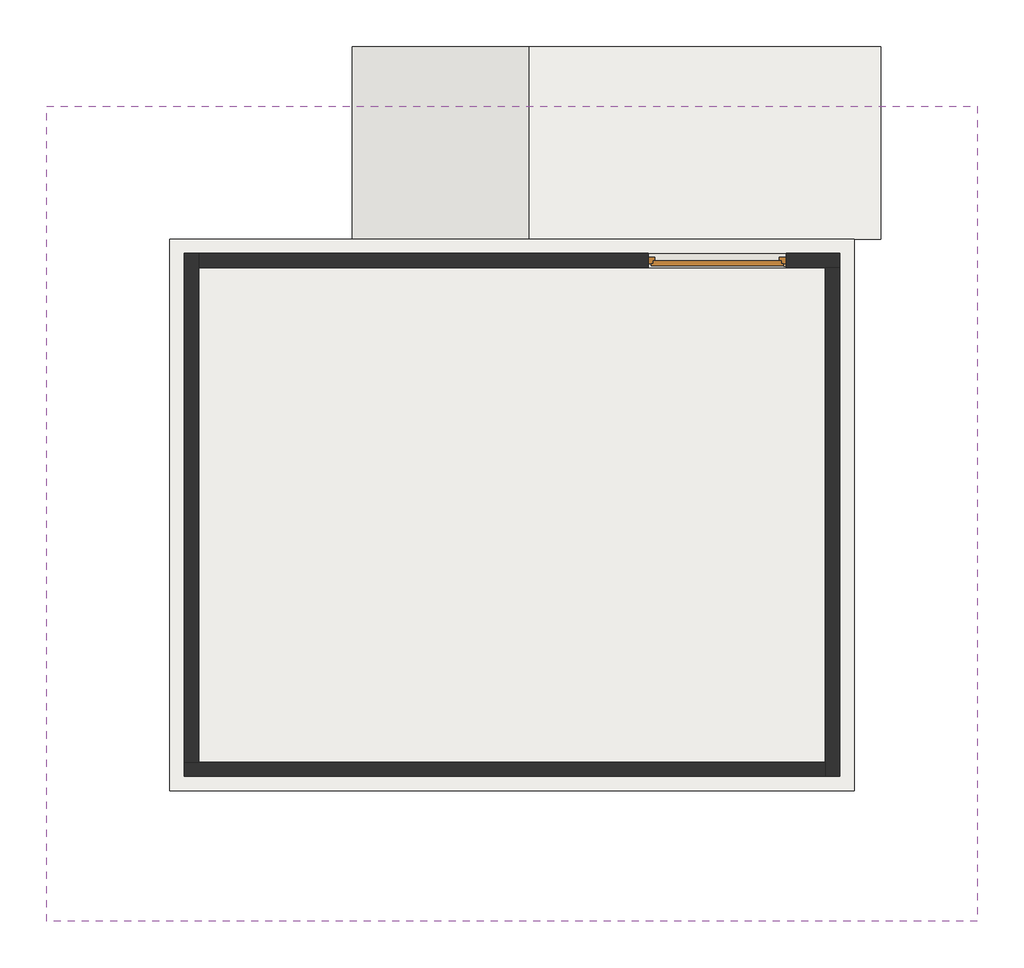
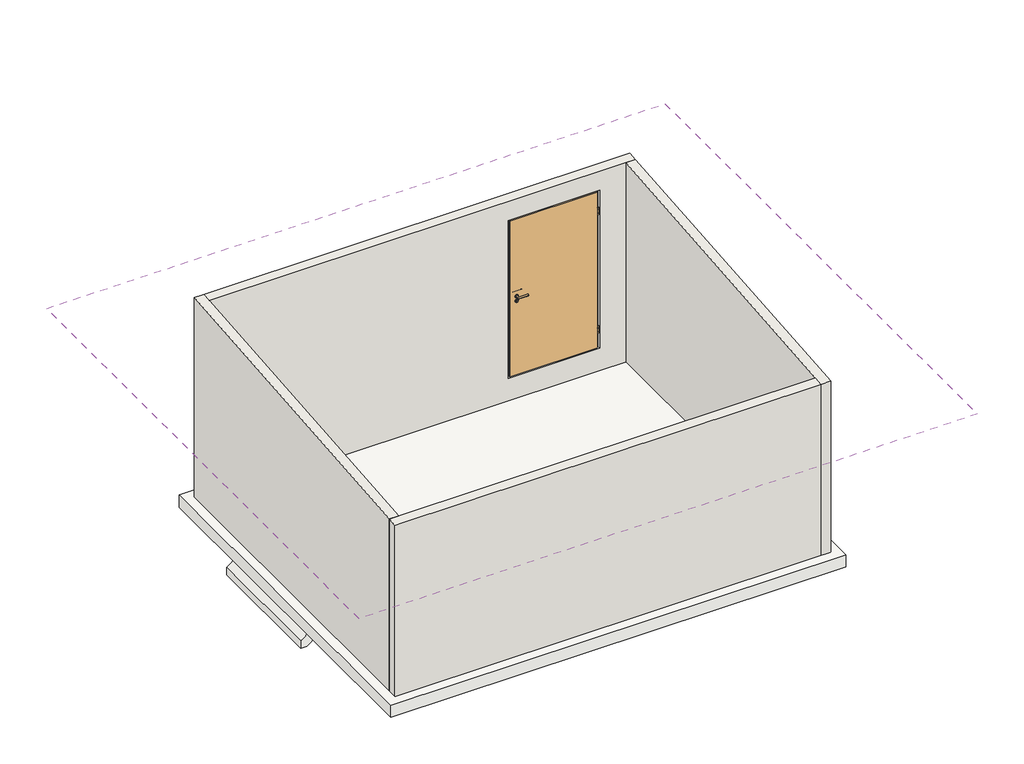
# One storey: 4 walls, 2 roofs, 1 door, 1 slab.
"""IFC4 building model written with IfcOpenShell, lengths in millimetres."""

import ifcopenshell
import ifcopenshell.guid

model = None  # the IFC model being written
_history = None  # IfcOwnerHistory: only IFC2X3 demands one
_inside = {}  # id of a spatial element -> (the spatial element, [elements in it])
_under = {}  # id of a project, library or spatial element -> (it, [spatial elements below it])
_declared = {}  # id of a project -> (the project, [libraries it declares])
_typed = {}  # id of a type object -> (the type object, [elements of that type])
_made_of = {}  # id of a material, layer set ... -> (it, [elements and type objects made of it])


def new_model(schema):
    """Start an empty IFC model of exactly this schema.

    Asked for "IFC4X3", IfcOpenShell would pick the latest addendum, in which some entities
    have other attributes; the version numbers below select the first issue.
    IFC2X3 requires an IfcOwnerHistory on every rooted entity: one is made here for all.
    """
    global model, _history
    if schema == "IFC4X3":
        model = ifcopenshell.file(schema_version=(4, 3, 0, 0))
    else:
        model = ifcopenshell.file(schema=schema)
    _inside.clear()
    _under.clear()
    _declared.clear()
    _typed.clear()
    _made_of.clear()
    _history = None
    if model.schema == "IFC2X3":
        org = make("IfcOrganization", Name="unknown")
        user = make(
            "IfcPersonAndOrganization",
            ThePerson=make("IfcPerson", FamilyName="unknown"),
            TheOrganization=org,
        )
        app = make(
            "IfcApplication",
            ApplicationDeveloper=org,
            Version="unknown",
            ApplicationFullName="unknown",
            ApplicationIdentifier="unknown",
        )
        _history = make(
            "IfcOwnerHistory",
            OwningUser=user,
            OwningApplication=app,
            ChangeAction="ADDED",
            CreationDate=0,
        )
    return model


def make(cls, **values):
    """One entity of the class cls with the attributes given. An attribute that is None is left unset."""
    return model.create_entity(
        cls, **{name: value for name, value in values.items() if value is not None}
    )


def rooted(cls, **values):
    """An entity with a GlobalId (a new one), such as an element, a storey or a relation."""
    return make(cls, GlobalId=ifcopenshell.guid.new(), OwnerHistory=_history, **values)


def si_unit(unit_type, name, prefix=None):
    """IfcSIUnit, for example si_unit("LENGTHUNIT", "METRE", prefix="MILLI")."""
    return make("IfcSIUnit", UnitType=unit_type, Prefix=prefix, Name=name)


def assignment(units):
    """IfcUnitAssignment: the units of a project."""
    return None if units is None else make("IfcUnitAssignment", Units=units)


def point(xyz):
    """IfcCartesianPoint."""
    return None if xyz is None else make("IfcCartesianPoint", Coordinates=xyz)


def direction(xyz):
    """IfcDirection."""
    return None if xyz is None else make("IfcDirection", DirectionRatios=xyz)


def frame(location, z_axis=None, x_axis=None):
    """IfcAxis2Placement3D, a coordinate frame: its origin and axes. An axis left out is left unset."""
    return make(
        "IfcAxis2Placement3D",
        Location=point(location),
        Axis=direction(z_axis),
        RefDirection=direction(x_axis),
    )


def frame_2d(location, x_axis=None):
    """IfcAxis2Placement2D, a coordinate frame in the plane: its origin and x axis."""
    return make(
        "IfcAxis2Placement2D", Location=point(location), RefDirection=direction(x_axis)
    )


def origin():
    """The frame at (0, 0, 0) with its axes left unset."""
    return frame((0.0, 0.0, 0.0))


def place(relative_to, where):
    """IfcLocalPlacement: puts the frame where relative to a parent placement (None: the world)."""
    return make(
        "IfcLocalPlacement", PlacementRelTo=relative_to, RelativePlacement=where
    )


def context(
    kind, dimensions, precision=None, world=None, true_north=None, identifier=None
):
    """IfcGeometricRepresentationContext, for example the 3D "Model" context."""
    return make(
        "IfcGeometricRepresentationContext",
        ContextIdentifier=identifier,
        ContextType=kind,
        CoordinateSpaceDimension=dimensions,
        Precision=precision,
        WorldCoordinateSystem=world,
        TrueNorth=true_north,
    )


def project(units=None, contexts=None):
    """IfcProject with its units and contexts."""
    return rooted(
        "IfcProject",
        Name="project",
        RepresentationContexts=contexts,
        UnitsInContext=assignment(units),
    )


def spatial(cls, under=None, at=None, **own):
    """A site, building, storey or space (cls), placed at a placement, below another one or the project."""
    s = rooted(cls, ObjectPlacement=at, **own)
    if under is not None:
        _under.setdefault(under.id(), (under, []))[1].append(s)
    return s


def polyline(points):
    """IfcPolyline through the points."""
    return make("IfcPolyline", Points=[point(p) for p in points])


def circle_curve(where, radius):
    """IfcCircle in the frame where."""
    return make("IfcCircle", Position=where, Radius=radius)


def ellipse_curve(where, semi_axis1, semi_axis2):
    """IfcEllipse in the frame where."""
    return make(
        "IfcEllipse", Position=where, SemiAxis1=semi_axis1, SemiAxis2=semi_axis2
    )


def trimmed(basis, trim1, trim2, sense, master):
    """IfcTrimmedCurve: the piece of a basis curve between two trims."""
    return make(
        "IfcTrimmedCurve",
        BasisCurve=basis,
        Trim1=trim1,
        Trim2=trim2,
        SenseAgreement=sense,
        MasterRepresentation=master,
    )


def segment(curve, same_sense, transition):
    """IfcCompositeCurveSegment."""
    return make(
        "IfcCompositeCurveSegment",
        Transition=transition,
        SameSense=same_sense,
        ParentCurve=curve,
    )


def composite_curve(segments, self_intersect=None):
    """IfcCompositeCurve: segments joined end to end."""
    return make("IfcCompositeCurve", Segments=segments, SelfIntersect=self_intersect)


def outline(outer, holes=None, kind="AREA"):
    """IfcArbitraryClosedProfileDef: a profile drawn as a closed curve; with holes, ...WithVoids."""
    if holes is None:
        return make("IfcArbitraryClosedProfileDef", ProfileType=kind, OuterCurve=outer)
    return make(
        "IfcArbitraryProfileDefWithVoids",
        ProfileType=kind,
        OuterCurve=outer,
        InnerCurves=holes,
    )


def extrude(swept, where, along, depth):
    """IfcExtrudedAreaSolid: the profile swept, set in the frame where, extruded along a direction by depth."""
    return make(
        "IfcExtrudedAreaSolid",
        SweptArea=swept,
        Position=where,
        ExtrudedDirection=direction(along),
        Depth=depth,
    )


def faces_of(points, faces, orient=None, outer=None):
    """IfcFace entities. A face is a list of loops; a loop is a list of indices into points, from 0.

    orient and outer hold one flag for each loop. By default every Orientation is true, the
    first loop of a face is its IfcFaceOuterBound and the others are IfcFaceBound.
    """
    made = []
    for i, loops in enumerate(faces):
        bounds = []
        for j, loop in enumerate(loops):
            is_outer = j == 0 if outer is None else outer[i][j]
            bounds.append(
                make(
                    "IfcFaceOuterBound" if is_outer else "IfcFaceBound",
                    Bound=make("IfcPolyLoop", Polygon=[points[k] for k in loop]),
                    Orientation=True if orient is None else orient[i][j],
                )
            )
        made.append(make("IfcFace", Bounds=bounds))
    return made


def faceted_brep(points, faces, orient=None, outer=None, voids=None):
    """IfcFacetedBrep: a solid bounded by flat faces; with voids (closed shells), ...WithVoids."""
    shared = [point(p) for p in points]
    hull = make("IfcClosedShell", CfsFaces=faces_of(shared, faces, orient, outer))
    if voids is None:
        return make("IfcFacetedBrep", Outer=hull)
    return make(
        "IfcFacetedBrepWithVoids",
        Outer=hull,
        Voids=[
            make(cls, CfsFaces=faces_of(shared, fs, o, b)) for cls, fs, o, b in voids
        ],
    )


def shape(context_of_items, identifier, shape_type, items):
    """IfcShapeRepresentation: the items that make up one representation, for example the "Body"."""
    return make(
        "IfcShapeRepresentation",
        ContextOfItems=context_of_items,
        RepresentationIdentifier=identifier,
        RepresentationType=shape_type,
        Items=items,
    )


def source(mapping_origin, context_of_items, identifier, shape_type, items):
    """IfcRepresentationMap: a shape defined once, which mapped items show again and again."""
    return make(
        "IfcRepresentationMap",
        MappingOrigin=mapping_origin,
        MappedRepresentation=shape(context_of_items, identifier, shape_type, items),
    )


def transform(
    local_origin,
    x_axis=None,
    y_axis=None,
    z_axis=None,
    scale=None,
    scale2=None,
    scale3=None,
    uniform=True,
):
    """IfcCartesianTransformationOperator3D, or its non-uniform kind. x_axis, y_axis, z_axis: its Axis1, 2, 3."""
    if uniform:
        return make(
            "IfcCartesianTransformationOperator3D",
            Axis1=direction(x_axis),
            Axis2=direction(y_axis),
            LocalOrigin=point(local_origin),
            Scale=scale,
            Axis3=direction(z_axis),
        )
    return make(
        "IfcCartesianTransformationOperator3DnonUniform",
        Axis1=direction(x_axis),
        Axis2=direction(y_axis),
        LocalOrigin=point(local_origin),
        Scale=scale,
        Axis3=direction(z_axis),
        Scale2=scale2,
        Scale3=scale3,
    )


def mapped(mapping_source, mapping_target):
    """IfcMappedItem: shows the shape of a source again, moved by a transform."""
    return make(
        "IfcMappedItem", MappingSource=mapping_source, MappingTarget=mapping_target
    )


def made_of(thing, what):
    """Note that an element or type object is made of a material, layer set ...; save() writes the relation."""
    if what is not None:
        _made_of.setdefault(what.id(), (what, []))[1].append(thing)
    return thing


def element(
    cls,
    number,
    at=None,
    inside=None,
    cuts=None,
    type_object=None,
    material=None,
    context=None,
    identifier="Body",
    shape_type=None,
    held_by="IfcProductDefinitionShape",
    body=None,
    shapes=None,
    **own,
):
    """One element of the class cls, such as IfcWall. Its Tag is "e" and its number.

    at: its placement. inside: the storey or other place that contains it. cuts: it is an
    opening in that element (IfcRelVoidsElement). A single representation is given by context,
    identifier, shape_type and body (its items); several are given by shapes. held_by: the class
    of the entity that holds the representations. save() writes the other relations.
    """
    e = rooted(cls, Tag="e%d" % number, ObjectPlacement=at, **own)
    if body is not None:
        shapes = [shape(context, identifier, shape_type, body)]
    if shapes is not None:
        e.Representation = make(held_by, Representations=shapes)
    if inside is not None:
        _inside.setdefault(inside.id(), (inside, []))[1].append(e)
    if cuts is not None:
        rooted(
            "IfcRelVoidsElement", RelatingBuildingElement=cuts, RelatedOpeningElement=e
        )
    if type_object is not None:
        _typed.setdefault(type_object.id(), (type_object, []))[1].append(e)
    return made_of(e, material)


def aggregate(whole, parts):
    """IfcRelAggregates: a whole, such as a stair, and the parts it consists of."""
    return rooted("IfcRelAggregates", RelatingObject=whole, RelatedObjects=parts)


def save(model, path):
    """Write the relations noted so far, then the file.

    IfcRelAggregates (storeys below a building ...), IfcRelContainedInSpatialStructure (elements
    in a storey), IfcRelDefinesByType, IfcRelAssociatesMaterial and IfcRelDeclares: one each for
    every whole, place, type object, material and project.
    """
    for whole, parts in _under.values():
        aggregate(whole, parts)
    for where, things in _inside.values():
        rooted(
            "IfcRelContainedInSpatialStructure",
            RelatedElements=things,
            RelatingStructure=where,
        )
    for kind, things in _typed.values():
        rooted("IfcRelDefinesByType", RelatedObjects=things, RelatingType=kind)
    for what, things in _made_of.values():
        rooted("IfcRelAssociatesMaterial", RelatedObjects=things, RelatingMaterial=what)
    for by, libraries in _declared.values():
        rooted("IfcRelDeclares", RelatingContext=by, RelatedDefinitions=libraries)
    model.write(path)


def plane_surface(at):
    """IfcPlane: the flat surface through the origin of the frame at, square to its z axis."""
    return make("IfcPlane", Position=at)


def cylinder_surface(at, radius):
    """IfcCylindricalSurface: all points at the distance radius from the z axis of the frame at."""
    return make("IfcCylindricalSurface", Position=at, Radius=radius)


def advanced_brep(points, edges, surfaces, faces):
    """IfcAdvancedBrep: a solid bounded by faces that lie on surfaces and meet in shared edges.

    An edge is (start, end): straight between two places in points (the first is 0);
    or (start, end, curve); or (start, end, curve, False) where it runs against its curve.
    A face is (place in surfaces, loops), or (place, loops, False) where it looks against
    its surface's normal. A loop lists edges by number (the first is 1), with a minus sign
    where the edge is run from its end to its start. The first loop is the outer one.
    """
    corners = [point(p) for p in points]
    vertices = [make("IfcVertexPoint", VertexGeometry=c) for c in corners]
    made = []
    for start, end, *more in edges:
        made.append(
            make(
                "IfcEdgeCurve",
                EdgeStart=vertices[start],
                EdgeEnd=vertices[end],
                EdgeGeometry=more[0] if more else make("IfcPolyline", Points=[corners[start], corners[end]]),
                SameSense=more[1] if len(more) > 1 else True,
            )
        )
    hull = []
    for where, loops, *sense in faces:
        bounds = []
        for j, loop in enumerate(loops):
            ring = [make("IfcOrientedEdge", EdgeElement=made[abs(k) - 1], Orientation=k > 0) for k in loop]
            bounds.append(
                make(
                    "IfcFaceOuterBound" if j == 0 else "IfcFaceBound",
                    Bound=make("IfcEdgeLoop", EdgeList=ring),
                    Orientation=True,
                )
            )
        hull.append(make("IfcAdvancedFace", Bounds=bounds, FaceSurface=surfaces[where], SameSense=sense[0] if sense else True))
    return make("IfcAdvancedBrep", Outer=make("IfcClosedShell", CfsFaces=hull))


def ml_1150_x_2100_f64283a4(model_context):
    return source(origin(), model_context, "Body", "SolidModel", [
        faceted_brep([(550.0, -44.5, 0.0), (-550.0, -44.5, 0.0), (-550.0, -27.5, 0.0), (-535.0, -27.5, 0.0), (-535.0, 0.5, 0.0), (535.0, 0.5, 0.0), (535.0, -27.5, 0.0), (550.0, -27.5, 0.0), (550.0, -44.5, 2075.0), (-550.0, -44.5, 2075.0), (-550.0, -27.5, 2075.0), (-535.0, -27.5, 2060.0), (550.0, -27.5, 2075.0), (535.0, -27.5, 2060.0), (-535.0, 0.5, 2060.0), (535.0, 0.5, 2060.0)], [[[0, 1, 2, 3, 4, 5, 6, 7]], [[8, 9, 1, 0]], [[1, 9, 10, 2]], [[11, 3, 2, 10, 12, 7, 6, 13]], [[3, 11, 14, 4]], [[5, 4, 14, 15]], [[13, 6, 5, 15]], [[8, 0, 7, 12]], [[9, 8, 12, 10]], [[11, 13, 15, 14]]]),
        extrude(outline(composite_curve([segment(trimmed(circle_curve(frame_2d((562.0, -37.5)), 10.0), [point((552.0, -37.5))], [point((572.0, -37.5))], False, "CARTESIAN"), True, "CONTINUOUS"), segment(trimmed(circle_curve(frame_2d((562.0, -37.5)), 10.0), [point((572.0, -37.5))], [point((552.0, -37.5))], False, "CARTESIAN"), True, "CONTINUOUS")], self_intersect=False)), frame((0.0, 0.0, 1844.0), z_axis=(0.0, 0.0, 1.0), x_axis=(1.0, 0.0, 0.0)), (0.0, 0.0, 1.0), 25.0),
        extrude(outline(composite_curve([segment(trimmed(circle_curve(frame_2d((562.0, -37.5)), 10.0), [point((562.0, -27.5))], [point((553.339746, -32.5))], False, "CARTESIAN"), True, "CONTINUOUS"), segment(polyline([(553.339746, -32.5), (550.0, -32.5), (550.0, -27.5), (562.0, -27.5)]), True, "CONTINUOUS")], self_intersect=False)), frame((0.0, 0.0, 1794.0), z_axis=(0.0, 0.0, 1.0), x_axis=(1.0, 0.0, 0.0)), (0.0, 0.0, 1.0), 50.0),
        extrude(outline(composite_curve([segment(trimmed(circle_curve(frame_2d((562.0, -37.5)), 10.0), [point((552.0, -37.5))], [point((572.0, -37.5))], False, "CARTESIAN"), True, "CONTINUOUS"), segment(trimmed(circle_curve(frame_2d((562.0, -37.5)), 10.0), [point((572.0, -37.5))], [point((552.0, -37.5))], False, "CARTESIAN"), True, "CONTINUOUS")], self_intersect=False)), frame((0.0, 0.0, 1769.0), z_axis=(0.0, 0.0, 1.0), x_axis=(1.0, 0.0, 0.0)), (0.0, 0.0, 1.0), 25.0),
        extrude(outline(composite_curve([segment(trimmed(circle_curve(frame_2d((562.0, -37.5)), 10.0), [point((552.0, -37.5))], [point((572.0, -37.5))], False, "CARTESIAN"), True, "CONTINUOUS"), segment(trimmed(circle_curve(frame_2d((562.0, -37.5)), 10.0), [point((572.0, -37.5))], [point((552.0, -37.5))], False, "CARTESIAN"), True, "CONTINUOUS")], self_intersect=False)), frame((0.0, 0.0, 266.0), z_axis=(0.0, 0.0, 1.0), x_axis=(1.0, 0.0, 0.0)), (0.0, 0.0, 1.0), 25.0),
        extrude(outline(composite_curve([segment(trimmed(circle_curve(frame_2d((562.0, -37.5)), 10.0), [point((562.0, -27.5))], [point((553.339746, -32.5))], False, "CARTESIAN"), True, "CONTINUOUS"), segment(polyline([(553.339746, -32.5), (550.0, -32.5), (550.0, -27.5), (562.0, -27.5)]), True, "CONTINUOUS")], self_intersect=False)), frame((0.0, 0.0, 216.0), z_axis=(0.0, 0.0, 1.0), x_axis=(1.0, 0.0, 0.0)), (0.0, 0.0, 1.0), 50.0),
        extrude(outline(composite_curve([segment(trimmed(circle_curve(frame_2d((562.0, -37.5)), 10.0), [point((552.0, -37.5))], [point((572.0, -37.5))], False, "CARTESIAN"), True, "CONTINUOUS"), segment(trimmed(circle_curve(frame_2d((562.0, -37.5)), 10.0), [point((572.0, -37.5))], [point((552.0, -37.5))], False, "CARTESIAN"), True, "CONTINUOUS")], self_intersect=False)), frame((0.0, 0.0, 191.0), z_axis=(0.0, 0.0, 1.0), x_axis=(1.0, 0.0, 0.0)), (0.0, 0.0, 1.0), 25.0),
        advanced_brep(
        [(-455.0, -54.5, 1050.0), (-475.0, -54.5, 1050.0), (-475.0, -104.5, 1050.0), (-455.0, -84.5, 1050.0), (-345.0, -84.5, 1050.0), (-345.0, -104.5, 1050.0)],
        [
            (0, 1, circle_curve(frame((-465.0, -54.5, 1050.0), z_axis=(0.0, 1.0, 0.0), x_axis=(-1.0, 0.0, 0.0)), 10.0)),
            (1, 0, circle_curve(frame((-465.0, -54.5, 1050.0), z_axis=(0.0, 1.0, 0.0), x_axis=(-1.0, 0.0, 0.0)), 10.0)),
            (1, 2),
            (2, 3, ellipse_curve(frame((-465.0, -94.5, 1050.0), z_axis=(-0.7071067811865531, 0.7071067811865419, 0.0), x_axis=(0.707106781186542, 0.707106781186553, 0.0)), 14.1421356, 10.0)),
            (3, 0),
            (3, 2, ellipse_curve(frame((-465.0, -94.5, 1050.0), z_axis=(-0.7071067811865531, 0.7071067811865419, 0.0), x_axis=(0.707106781186542, 0.707106781186553, 0.0)), 14.1421356, 10.0)),
            (4, 5, circle_curve(frame((-345.0, -94.5, 1050.0), z_axis=(1.0, 0.0, 0.0), x_axis=(0.0, -1.0, 0.0)), 10.0)),
            (5, 4, circle_curve(frame((-345.0, -94.5, 1050.0), z_axis=(1.0, 0.0, 0.0), x_axis=(0.0, -1.0, 0.0)), 10.0)),
            (2, 5),
            (4, 3),
        ],
        [
            plane_surface(frame((-465.0, -54.5, 1050.0), z_axis=(0.0, 1.0, 0.0), x_axis=(0.0, 0.0, 1.0))),
            cylinder_surface(frame((-465.0, -54.5, 1050.0), z_axis=(0.0, 1.0, 0.0), x_axis=(-1.0, 0.0, 0.0)), 10.0),
            plane_surface(frame((-345.0, -94.5, 1050.0), z_axis=(1.0, 0.0, 0.0), x_axis=(0.0, 0.0, 1.0))),
            cylinder_surface(frame((-465.0, -94.5, 1050.0), z_axis=(-1.0, 0.0, 0.0), x_axis=(0.0, -1.0, 0.0)), 10.0),
        ],
        [
            (0, [[1, 2]]),
            (1, [[3, 4, 5, -2]]),
            (1, [[-5, 6, -3, -1]]),
            (2, [[7, 8]]),
            (3, [[9, -7, 10, -4]]),
            (3, [[-10, -8, -9, -6]]),
        ],
    ),
        extrude(outline(composite_curve([segment(trimmed(circle_curve(frame_2d((990.0, -465.0)), 20.0), [point((990.0, -485.0))], [point((990.0, -445.0))], False, "CARTESIAN"), True, "CONTINUOUS"), segment(trimmed(circle_curve(frame_2d((990.0, -465.0)), 20.0), [point((990.0, -445.0))], [point((990.0, -485.0))], False, "CARTESIAN"), True, "CONTINUOUS")], self_intersect=False), holes=[composite_curve([segment(polyline([(976.4601385, -467.397268), (988.4749012, -467.397268)]), True, "CONTINUOUS"), segment(trimmed(circle_curve(frame_2d((995.0361633, -465.0)), 6.9854888), [point((988.4749012, -467.397268))], [point((988.4749012, -462.602732))], True, "CARTESIAN"), True, "CONTINUOUS"), segment(polyline([(988.4749012, -462.602732), (976.4601385, -462.602732)]), True, "CONTINUOUS"), segment(trimmed(circle_curve(frame_2d((976.4601385, -465.0)), 2.397268), [point((976.4601385, -462.602732))], [point((976.4601385, -467.397268))], True, "CARTESIAN"), True, "CONTINUOUS")], self_intersect=False)]), frame((0.0, -54.5, 0.0), z_axis=(0.0, 1.0, 0.0), x_axis=(0.0, 0.0, 1.0)), (0.0, 0.0, 1.0), 10.0),
        advanced_brep(
        [(-455.0, -54.5, 1050.0), (-475.0, -54.5, 1050.0), (-475.0, -104.5, 1050.0), (-455.0, -84.5, 1050.0), (-345.0, -84.5, 1050.0), (-345.0, -104.5, 1050.0)],
        [
            (0, 1, circle_curve(frame((-465.0, -54.5, 1050.0), z_axis=(0.0, 1.0, 0.0), x_axis=(-1.0, 0.0, 0.0)), 10.0)),
            (1, 0, circle_curve(frame((-465.0, -54.5, 1050.0), z_axis=(0.0, 1.0, 0.0), x_axis=(-1.0, 0.0, 0.0)), 10.0)),
            (1, 2),
            (2, 3, ellipse_curve(frame((-465.0, -94.5, 1050.0), z_axis=(-0.7071067811865537, 0.7071067811865414, 0.0), x_axis=(0.7071067811865414, 0.7071067811865536, 0.0)), 14.1421356, 10.0)),
            (3, 0),
            (3, 2, ellipse_curve(frame((-465.0, -94.5, 1050.0), z_axis=(-0.7071067811865537, 0.7071067811865414, 0.0), x_axis=(0.7071067811865414, 0.7071067811865536, 0.0)), 14.1421356, 10.0)),
            (4, 5, circle_curve(frame((-345.0, -94.5, 1050.0), z_axis=(1.0, 0.0, 0.0), x_axis=(0.0, -1.0, 0.0)), 10.0)),
            (5, 4, circle_curve(frame((-345.0, -94.5, 1050.0), z_axis=(1.0, 0.0, 0.0), x_axis=(0.0, -1.0, 0.0)), 10.0)),
            (2, 5),
            (4, 3),
        ],
        [
            plane_surface(frame((-465.0, -54.5, 1050.0), z_axis=(0.0, 1.0, 0.0), x_axis=(0.0, 0.0, 1.0))),
            cylinder_surface(frame((-465.0, -54.5, 1050.0), z_axis=(0.0, 1.0, 0.0), x_axis=(-1.0, 0.0, 0.0)), 10.0),
            plane_surface(frame((-345.0, -94.5, 1050.0), z_axis=(1.0, 0.0, 0.0), x_axis=(0.0, 0.0, 1.0))),
            cylinder_surface(frame((-465.0, -94.5, 1050.0), z_axis=(-1.0, 0.0, 0.0), x_axis=(0.0, -1.0, 0.0)), 10.0),
        ],
        [
            (0, [[1, 2]]),
            (1, [[3, 4, 5, -2]]),
            (1, [[-5, 6, -3, -1]]),
            (2, [[7, 8]]),
            (3, [[9, -7, 10, -4]]),
            (3, [[-10, -8, -9, -6]]),
        ],
    ),
        extrude(outline(composite_curve([segment(trimmed(circle_curve(frame_2d((1050.0, -465.0)), 20.0), [point((1050.0, -485.0))], [point((1050.0, -445.0))], False, "CARTESIAN"), True, "CONTINUOUS"), segment(trimmed(circle_curve(frame_2d((1050.0, -465.0)), 20.0), [point((1050.0, -445.0))], [point((1050.0, -485.0))], False, "CARTESIAN"), True, "CONTINUOUS")], self_intersect=False)), frame((0.0, -54.5, 0.0), z_axis=(0.0, 1.0, 0.0), x_axis=(0.0, 0.0, 1.0)), (0.0, 0.0, 1.0), 10.0),
        advanced_brep(
        [(-455.0, 10.5, 1050.0), (-475.0, 10.5, 1050.0), (-455.0, 40.5, 1050.0), (-475.0, 60.5, 1050.0), (-345.0, 40.5, 1050.0), (-345.0, 60.5, 1050.0)],
        [
            (0, 1, circle_curve(frame((-465.0, 10.5, 1050.0), z_axis=(0.0, -1.0, 0.0), x_axis=(-1.0, 0.0, 0.0)), 10.0)),
            (1, 0, circle_curve(frame((-465.0, 10.5, 1050.0), z_axis=(0.0, -1.0, 0.0), x_axis=(-1.0, 0.0, 0.0)), 10.0)),
            (0, 2),
            (2, 3, ellipse_curve(frame((-465.0, 50.5, 1050.0), z_axis=(-0.7071067811865486, -0.7071067811865464, 0.0), x_axis=(0.7071067811865464, -0.7071067811865488, 0.0)), 14.1421356, 10.0)),
            (3, 1),
            (3, 2, ellipse_curve(frame((-465.0, 50.5, 1050.0), z_axis=(-0.7071067811865486, -0.7071067811865464, 0.0), x_axis=(0.7071067811865464, -0.7071067811865488, 0.0)), 14.1421356, 10.0)),
            (4, 5, circle_curve(frame((-345.0, 50.5, 1050.0), z_axis=(1.0, 0.0, 0.0), x_axis=(0.0, 1.0, 0.0)), 10.0)),
            (5, 4, circle_curve(frame((-345.0, 50.5, 1050.0), z_axis=(1.0, 0.0, 0.0), x_axis=(0.0, 1.0, 0.0)), 10.0)),
            (2, 4),
            (5, 3),
        ],
        [
            plane_surface(frame((-465.0, 10.5, 1050.0), z_axis=(0.0, -1.0, 0.0), x_axis=(0.0, 0.0, 1.0))),
            cylinder_surface(frame((-465.0, 10.5, 1050.0), z_axis=(0.0, -1.0, 0.0), x_axis=(-1.0, 0.0, 0.0)), 10.0),
            plane_surface(frame((-345.0, 50.5, 1050.0), z_axis=(1.0, 0.0, 0.0), x_axis=(0.0, 0.0, 1.0))),
            cylinder_surface(frame((-465.0, 50.5, 1050.0), z_axis=(-1.0, 0.0, 0.0), x_axis=(0.0, 1.0, 0.0)), 10.0),
        ],
        [
            (0, [[1, 2]]),
            (1, [[-1, 3, 4, 5]]),
            (1, [[-2, -5, 6, -3]]),
            (2, [[7, 8]]),
            (3, [[-4, 9, -8, 10]]),
            (3, [[-6, -10, -7, -9]]),
        ],
    ),
        extrude(outline(composite_curve([segment(trimmed(circle_curve(frame_2d((990.0, -465.0)), 20.0), [point((990.0, -485.0))], [point((990.0, -445.0))], False, "CARTESIAN"), True, "CONTINUOUS"), segment(trimmed(circle_curve(frame_2d((990.0, -465.0)), 20.0), [point((990.0, -445.0))], [point((990.0, -485.0))], False, "CARTESIAN"), True, "CONTINUOUS")], self_intersect=False), holes=[composite_curve([segment(polyline([(976.4601385, -467.397268), (988.4749012, -467.397268)]), True, "CONTINUOUS"), segment(trimmed(circle_curve(frame_2d((995.0361633, -465.0)), 6.9854888), [point((988.4749012, -467.397268))], [point((988.4749012, -462.602732))], True, "CARTESIAN"), True, "CONTINUOUS"), segment(polyline([(988.4749012, -462.602732), (976.4601385, -462.602732)]), True, "CONTINUOUS"), segment(trimmed(circle_curve(frame_2d((976.4601385, -465.0)), 2.397268), [point((976.4601385, -462.602732))], [point((976.4601385, -467.397268))], True, "CARTESIAN"), True, "CONTINUOUS")], self_intersect=False)]), frame((0.0, 0.5, 0.0), z_axis=(0.0, 1.0, 0.0), x_axis=(0.0, 0.0, 1.0)), (0.0, 0.0, 1.0), 10.0),
        advanced_brep(
        [(-455.0, 10.5, 1050.0), (-475.0, 10.5, 1050.0), (-455.0, 40.5, 1050.0), (-475.0, 60.5, 1050.0), (-345.0, 40.5, 1050.0), (-345.0, 60.5, 1050.0)],
        [
            (0, 1, circle_curve(frame((-465.0, 10.5, 1050.0), z_axis=(0.0, -1.0, 0.0), x_axis=(-1.0, 0.0, 0.0)), 10.0)),
            (1, 0, circle_curve(frame((-465.0, 10.5, 1050.0), z_axis=(0.0, -1.0, 0.0), x_axis=(-1.0, 0.0, 0.0)), 10.0)),
            (0, 2),
            (2, 3, ellipse_curve(frame((-465.0, 50.5, 1050.0), z_axis=(-0.7071067811865491, -0.7071067811865459, 0.0), x_axis=(0.7071067811865458, -0.7071067811865492, 0.0)), 14.1421356, 10.0)),
            (3, 1),
            (3, 2, ellipse_curve(frame((-465.0, 50.5, 1050.0), z_axis=(-0.7071067811865491, -0.7071067811865459, 0.0), x_axis=(0.7071067811865458, -0.7071067811865492, 0.0)), 14.1421356, 10.0)),
            (4, 5, circle_curve(frame((-345.0, 50.5, 1050.0), z_axis=(1.0, 0.0, 0.0), x_axis=(0.0, 1.0, 0.0)), 10.0)),
            (5, 4, circle_curve(frame((-345.0, 50.5, 1050.0), z_axis=(1.0, 0.0, 0.0), x_axis=(0.0, 1.0, 0.0)), 10.0)),
            (2, 4),
            (5, 3),
        ],
        [
            plane_surface(frame((-465.0, 10.5, 1050.0), z_axis=(0.0, -1.0, 0.0), x_axis=(0.0, 0.0, 1.0))),
            cylinder_surface(frame((-465.0, 10.5, 1050.0), z_axis=(0.0, -1.0, 0.0), x_axis=(-1.0, 0.0, 0.0)), 10.0),
            plane_surface(frame((-345.0, 50.5, 1050.0), z_axis=(1.0, 0.0, 0.0), x_axis=(0.0, 0.0, 1.0))),
            cylinder_surface(frame((-465.0, 50.5, 1050.0), z_axis=(-1.0, 0.0, 0.0), x_axis=(0.0, 1.0, 0.0)), 10.0),
        ],
        [
            (0, [[1, 2]]),
            (1, [[-1, 3, 4, 5]]),
            (1, [[-2, -5, 6, -3]]),
            (2, [[7, 8]]),
            (3, [[-4, 9, -8, 10]]),
            (3, [[-6, -10, -7, -9]]),
        ],
    ),
        extrude(outline(composite_curve([segment(trimmed(circle_curve(frame_2d((1050.0, -465.0)), 20.0), [point((1050.0, -485.0))], [point((1050.0, -445.0))], False, "CARTESIAN"), True, "CONTINUOUS"), segment(trimmed(circle_curve(frame_2d((1050.0, -465.0)), 20.0), [point((1050.0, -445.0))], [point((1050.0, -485.0))], False, "CARTESIAN"), True, "CONTINUOUS")], self_intersect=False)), frame((0.0, 0.5, 0.0), z_axis=(0.0, 1.0, 0.0), x_axis=(0.0, 0.0, 1.0)), (0.0, 0.0, 1.0), 10.0),
        faceted_brep([(-535.0, -27.5, 0.0), (-575.0, -27.5, 0.0), (-575.0, 27.5, 0.0), (-520.0, 27.5, 0.0), (-520.0, 0.5, 0.0), (-535.0, 0.5, 0.0), (-535.0, 0.5, 2060.0), (-535.0, -27.5, 2060.0), (-520.0, 0.5, 2045.0), (520.0, 0.5, 2045.0), (520.0, 0.5, 0.0), (535.0, 0.5, 0.0), (535.0, 0.5, 2060.0), (-520.0, 27.5, 2045.0), (-575.0, 27.5, 2100.0), (575.0, 27.5, 2100.0), (575.0, 27.5, 0.0), (520.0, 27.5, 0.0), (520.0, 27.5, 2045.0), (-575.0, -27.5, 2100.0), (535.0, -27.5, 2060.0), (535.0, -27.5, 0.0), (575.0, -27.5, 0.0), (575.0, -27.5, 2100.0)], [[[0, 1, 2, 3, 4, 5]], [[5, 6, 7, 0]], [[4, 8, 9, 10, 11, 12, 6, 5]], [[3, 13, 8, 4]], [[2, 14, 15, 16, 17, 18, 13, 3]], [[1, 19, 14, 2]], [[0, 7, 20, 21, 22, 23, 19, 1]], [[23, 22, 16, 15]], [[21, 11, 10, 17, 16, 22]], [[12, 11, 21, 20]], [[18, 17, 10, 9]], [[19, 23, 15, 14]], [[13, 18, 9, 8]], [[6, 12, 20, 7]]]),
    ])


model = new_model("IFC4")

# Units and contexts
model_context = context("Model", 3, world=origin())
ifc_project = project(units=[si_unit("LENGTHUNIT", "METRE", prefix="MILLI")], contexts=[model_context])

# Site, building, storey
site = spatial("IfcSite", under=ifc_project)
building = spatial("IfcBuilding", under=site)
storey = spatial("IfcBuildingStorey", under=building, Name="OG1- OK RD", Elevation=3650.0)

# Door
placement = place(None, origin())
ml_1150_x_2100_shape = ml_1150_x_2100_f64283a4(model_context)
element("IfcDoor", 1, ObjectType="TU DF 1 - Pfostenstock Falztüre : ML - 1150 x 2100", at=placement, inside=storey, context=model_context, shape_type="MappedRepresentation", body=[
    mapped(ml_1150_x_2100_shape, transform((10907.9226469, 8574.5272422, 3950.0), x_axis=(1.0, 0.0, 0.0), y_axis=(0.0, 1.0, 0.0), z_axis=(0.0, 0.0, 1.0))),
])

# Roofs
element("IfcRoof", 2, ObjectType="Bitumendach_KLH 160_Bitumen 5_165", at=placement, inside=storey, context=model_context, shape_type="SweptSolid", body=[
    extrude(outline(polyline([(3054.5272422, 5989.3089419), (9864.5272422, 6585.1067405), (9864.5272422, 6419.4764673), (3054.5272422, 5823.6786687), (3054.5272422, 5989.3089419)])), frame((5302.9226469, 0.0, 0.0), z_axis=(1.0, 0.0, 0.0), x_axis=(0.0, 1.0, 0.0)), (0.0, 0.0, 1.0), 7780.0),
])
element("IfcRoof", 3, ObjectType="Bitumendach_KLH 120_Bitumenbahn 5_125", at=placement, inside=storey, context=model_context, shape_type="SweptSolid", body=[
    extrude(outline(polyline([(2295.0, 9332.0735765), (1175.9836286, 7859.6836823), (1075.9836286, 7859.6836823), (1075.9836286, 7934.6878727), (2170.0, 9374.1830316), (2170.0, 12272.9226469), (2295.0, 12272.9226469), (2295.0, 9332.0735765)])), frame((0.0, 8754.5272422, 0.0), z_axis=(0.0, 1.0, 0.0), x_axis=(0.0, 0.0, 1.0)), (0.0, 0.0, 1.0), 1610.0),
])

# Slab
element("IfcSlab", 4, ObjectType="KLH 160", at=placement, inside=storey, context=model_context, shape_type="SweptSolid", body=[
    extrude(outline(polyline([(12052.9226469, 4144.5272422), (6332.9226469, 4144.5272422), (6332.9226469, 8754.5272422), (12052.9226469, 8754.5272422), (12052.9226469, 4144.5272422)])), frame((0.0, 0.0, 3490.0), z_axis=(0.0, 0.0, 1.0), x_axis=(1.0, 0.0, 0.0)), (0.0, 0.0, 1.0), 160.0),
])

# Walls
element("IfcWall", 5, ObjectType="KLH 120", at=placement, inside=storey, context=model_context, shape_type="Brep", body=[
    faceted_brep([(6452.9226469, 4264.5272422, 3650.0), (11812.9226469, 4264.5272422, 3650.0), (11812.9226469, 4264.5272422, 5929.5399516), (6452.9226469, 4264.5272422, 5929.5399516), (6452.9226469, 4384.5272422, 3650.0), (6452.9226469, 4384.5272422, 5940.0385912), (6572.9226469, 4384.5272422, 5940.0385912), (11812.9226469, 4384.5272422, 5940.0385912), (11812.9226469, 4384.5272422, 3650.0), (6572.9226469, 4384.5272422, 3650.0)], [[[0, 1, 2, 3]], [[4, 5, 6, 7, 8, 9]], [[1, 0, 4, 9, 8]], [[0, 3, 5, 4]], [[2, 1, 8, 7]], [[3, 2, 7, 6, 5]]]),
])
element("IfcWall", 6, ObjectType="KLH 120", at=placement, inside=storey, context=model_context, shape_type="Brep", body=[
    faceted_brep([(6452.9226469, 8634.5272422, 3650.0), (6452.9226469, 4384.5272422, 3650.0), (6452.9226469, 4384.5272422, 5940.0385912), (6452.9226469, 8634.5272422, 6311.8654112), (6572.9226469, 8634.5272422, 3650.0), (6572.9226469, 8634.5272422, 6311.8654112), (6572.9226469, 8514.5272422, 6301.3667716), (6572.9226469, 4384.5272422, 5940.0385912), (6572.9226469, 4384.5272422, 3650.0), (6572.9226469, 8514.5272422, 3650.0)], [[[0, 1, 2, 3]], [[4, 5, 6, 7, 8, 9]], [[1, 0, 4, 9, 8]], [[2, 1, 8, 7]], [[0, 3, 5, 4]], [[3, 2, 7, 6, 5]]]),
])
element("IfcWall", 7, ObjectType="KLH 120", at=placement, inside=storey, context=model_context, shape_type="Brep", body=[
    faceted_brep([(11932.9226469, 8634.5272422, 3650.0), (6572.9226469, 8634.5272422, 3650.0), (6572.9226469, 8634.5272422, 6311.8654112), (11932.9226469, 8634.5272422, 6311.8654112), (11482.9226469, 8634.5272422, 6050.0), (10332.9226469, 8634.5272422, 6050.0), (10332.9226469, 8634.5272422, 3950.0), (11482.9226469, 8634.5272422, 3950.0), (11932.9226469, 8514.5272422, 3650.0), (11932.9226469, 8514.5272422, 6301.3667716), (11812.9226469, 8514.5272422, 6301.3667716), (6572.9226469, 8514.5272422, 6301.3667716), (6572.9226469, 8514.5272422, 3650.0), (11812.9226469, 8514.5272422, 3650.0), (11482.9226469, 8514.5272422, 6050.0), (11482.9226469, 8514.5272422, 3950.0), (10332.9226469, 8514.5272422, 3950.0), (10332.9226469, 8514.5272422, 6050.0)], [[[0, 1, 2, 3], [4, 5, 6, 7]], [[8, 9, 10, 11, 12, 13], [14, 15, 16, 17]], [[1, 0, 8, 13, 12]], [[2, 1, 12, 11]], [[0, 3, 9, 8]], [[3, 2, 11, 10, 9]], [[15, 14, 4, 7]], [[16, 15, 7, 6]], [[17, 16, 6, 5]], [[14, 17, 5, 4]]]),
])
element("IfcWall", 8, ObjectType="KLH 120", at=placement, inside=storey, context=model_context, shape_type="Brep", body=[
    faceted_brep([(11932.9226469, 4264.5272422, 3650.0), (11932.9226469, 8514.5272422, 3650.0), (11932.9226469, 8514.5272422, 6301.3667716), (11932.9226469, 4264.5272422, 5929.5399516), (11812.9226469, 4264.5272422, 3650.0), (11812.9226469, 4264.5272422, 5929.5399516), (11812.9226469, 4384.5272422, 5940.0385912), (11812.9226469, 8514.5272422, 6301.3667716), (11812.9226469, 8514.5272422, 3650.0), (11812.9226469, 4384.5272422, 3650.0)], [[[0, 1, 2, 3]], [[4, 5, 6, 7, 8, 9]], [[1, 0, 4, 9, 8]], [[0, 3, 5, 4]], [[2, 1, 8, 7]], [[3, 2, 7, 6, 5]]]),
])

save(model, "model.ifc")

# Revit data of these elements
# Project information
#   Bauherr = "AUTODESK"
#   Baustellenort = "BAUORT"
#   Baustellenstraße = "BAUSTRASSE 1"
#   Gerichtsbezirk = "GERICHTSBEZIRK"
#   Grundstücksnummer = "GR"
#   Katastralgemeinde = "KG"
#   Kundenadresse = "KUNDENSTRASSE 1"
#   Kundenort = "KUNDENORT"
#   Kundenzusatz = "KUNDENZUSATZ"
#   Kundentelefon = "0000-00000-1"
#   Einlagezahl = "123-45"
#   PrintManagerSettings = "<PrintManagerDS xmlns=\"http://tempuri.org/PrintManagerDS.xsd\">\n  <xs:schema id=\"PrintManagerDS\" targetNamespace=\"http://tempuri.org/PrintManagerDS.xsd\" xmlns:mstns=\"http://tempuri.org/PrintManagerDS.xsd\" xmlns=\"http://tempuri.org/PrintManagerDS.xsd\" xmlns:xs=\"http://www.w3.org/2001/XMLSchema\" xmlns:msdata=\"urn:schemas-microsoft-com:xml-msdata\" attributeFormDefault=\"qualified\" elementFormDefault=\"qualified\">\n    <xs:element name=\"PrintManagerDS\" msdata:IsDataSet=\"true\" msdata:UseCurrentLocale=\"true\">\n      <xs:complexType>\n        <xs:choice minOccurs=\"0\" maxOccurs=\"unbounded\">\n          <xs:element name=\"DruckEinstellungDT\">\n            <xs:complexType>\n              <xs:sequence>\n                <xs:element name=\"ID\" msdata:DataType=\"System.Guid, mscorlib, Version=4.0.0.0, Culture=neutral, PublicKeyToken=b77a5c561934e089\" msdata:AutoIncrementSeed=\"-1\" msdata:AutoIncrementStep=\"-1\" type=\"xs:string\" minOccurs=\"0\" />\n                <xs:element name=\"Name\" type=\"xs:string\" minOccurs=\"0\" />\n                <xs:element name=\"Beschreibung\" type=\"xs:string\" minOccurs=\"0\" />\n                <xs:element name=\"Kategorie\" type=\"xs:string\" minOccurs=\"0\" />\n                <xs:element name=\"PrinterName\" type=\"xs:string\" minOccurs=\"0\" />\n                <xs:element name=\"PrintToFile\" type=\"xs:boolean\" minOccurs=\"0\" />\n                <xs:element name=\"FileName\" type=\"xs:string\" minOccurs=\"0\" />\n                <xs:element name=\"ColorDepth\" type=\"xs:string\" minOccurs=\"0\" />\n                <xs:element name=\"HiddenLineViews\" type=\"xs:string\" minOccurs=\"0\" />\n                <xs:element name=\"HideCropBoundaries\" type=\"xs:boolean\" minOccurs=\"0\" />\n                <xs:element name=\"HideRefOrWorkPlanes\" type=\"xs:boolean\" minOccurs=\"0\" />\n                <xs:element name=\"HideScopeBoxes\" type=\"xs:boolean\" minOccurs=\"0\" />\n                <xs:element name=\"HideUnreferencedViewTags\" type=\"xs:boolean\" minOccurs=\"0\" />\n                <xs:element name=\"MarginType\" type=\"xs:string\" minOccurs=\"0\" />\n                <xs:element name=\"PageOrientation\" type=\"xs:string\" minOccurs=\"0\" />\n                <xs:element name=\"PaperPlacement\" type=\"xs:string\" minOccurs=\"0\" />\n                <xs:element name=\"PaperSize\" type=\"xs:string\" minOccurs=\"0\" />\n                <xs:element name=\"PaperSource\" type=\"xs:string\" minOccurs=\"0\" />\n                <xs:element name=\"RasterQuality\" type=\"xs:string\" minOccurs=\"0\" />\n                <xs:element name=\"ReplaceHalftoneWithThinLines\" type=\"xs:boolean\" minOccurs=\"0\" />\n                <xs:element name=\"UserDefinedMarginX\" type=\"xs:double\" minOccurs=\"0\" />\n                <xs:element name=\"UserDefinedMarginY\" type=\"xs:double\" minOccurs=\"0\" />\n                <xs:element name=\"ViewLinksInBlue\" type=\"xs:boolean\" minOccurs=\"0\" />\n                <xs:element name=\"Zoom\" type=\"xs:int\" minOccurs=\"0\" />\n                <xs:element name=\"ZoomType\" type=\"xs:string\" minOccurs=\"0\" />\n              </xs:sequence>\n            </xs:complexType>\n          </xs:element>\n          <xs:element name=\"DruckSatzDT\">\n            <xs:complexType>\n              <xs:sequence>\n                <xs:element name=\"ID\" msdata:DataType=\"System.Guid, mscorlib, Version=4.0.0.0, Culture=neutral, PublicKeyToken=b77a5c561934e089\" type=\"xs:string\" minOccurs=\"0\" />\n                <xs:element name=\"PlanID\" type=\"xs:string\" minOccurs=\"0\" />\n                <xs:element name=\"DruckEinstellungID\" msdata:DataType=\"System.Guid, mscorlib, Version=4.0.0.0, Culture=neutral, PublicKeyToken=b77a5c561934e089\" type=\"xs:string\" minOccurs=\"0\" />\n                <xs:element name=\"Name\" type=\"xs:string\" minOccurs=\"0\" />\n                <xs:element name=\"Beschreibung\" type=\"xs:string\" minOccurs=\"0\" />\n                <xs:element name=\"ParameterName\" type=\"xs:string\" minOccurs=\"0\" />\n                <xs:element name=\"File\" type=\"xs:string\" minOccurs=\"0\" />\n                <xs:element name=\"Path\" type=\"xs:string\" minOccurs=\"0\" />\n                <xs:element name=\"GenerateFileName\" type=\"xs:boolean\" minOccurs=\"0\" />\n                <xs:element name=\"Kategorie\" type=\"xs:string\" minOccurs=\"0\" />\n              </xs:sequence>\n            </xs:complexType>\n          </xs:element>\n          <xs:element name=\"DruckJobDT\">\n            <xs:complexType>\n              <xs:sequence>\n                <xs:element name=\"ID\" msdata:DataType=\"System.Guid, mscorlib, Version=4.0.0.0, Culture=neutral, PublicKeyToken=b77a5c561934e089\" type=\"xs:string\" minOccurs=\"0\" />\n                <xs:element name=\"DruckJobGruppeID\" msdata:DataType=\"System.Guid, mscorlib, Version=4.0.0.0, Culture=neutral, PublicKeyToken=b77a5c561934e089\" type=\"xs:string\" minOccurs=\"0\" />\n                <xs:element name=\"DruckSatzID\" msdata:DataType=\"System.Guid, mscorlib, Version=4.0.0.0, Culture=neutral, PublicKeyToken=b77a5c561934e089\" type=\"xs:string\" minOccurs=\"0\" />\n                <xs:element name=\"Anzahl\" type=\"xs:int\" minOccurs=\"0\" />\n              </xs:sequence>\n            </xs:complexType>\n          </xs:element>\n          <xs:element name=\"DruckJobGruppeDT\">\n            <xs:complexType>\n              <xs:sequence>\n                <xs:element name=\"ID\" msdata:DataType=\"System.Guid, mscorlib, Version=4.0.0.0, Culture=neutral, PublicKeyToken=b77a5c561934e089\" type=\"xs:string\" minOccurs=\"0\" />\n                <xs:element name=\"Name\" type=\"xs:string\" minOccurs=\"0\" />\n                <xs:element name=\"Beschreibung\" type=\"xs:string\" minOccurs=\"0\" />\n                <xs:element name=\"JobCount\" msdata:ReadOnly=\"true\" msdata:Expression=\"Count(Child(DruckJobGruppeDT_DruckJobDT).Anzahl)\" type=\"xs:int\" minOccurs=\"0\" />\n                <xs:element name=\"Kategorie\" type=\"xs:string\" minOccurs=\"0\" />\n              </xs:sequence>\n            </xs:complexType>\n          </xs:element>\n          <xs:element name=\"PrintSettingCategories\">\n            <xs:complexType>\n              <xs:sequence>\n                <xs:element name=\"CategoryName\" type=\"xs:string\" minOccurs=\"0\" />\n              </xs:sequence>\n            </xs:complexType>\n          </xs:element>\n          <xs:element name=\"PrintRecordCategories\">\n            <xs:complexType>\n              <xs:sequence>\n                <xs:element name=\"CategoryName\" type=\"xs:string\" />\n              </xs:sequence>\n            </xs:complexType>\n          </xs:element>\n          <xs:element name=\"JobGroupCategories\">\n            <xs:complexType>\n              <xs:sequence>\n                <xs:element name=\"CategoryName\" type=\"xs:string\" />\n              </xs:sequence>\n            </xs:complexType>\n          </xs:element>\n          <xs:element name=\"ExportSettingsDT\">\n            <xs:complexType>\n              <xs:sequence>\n                <xs:element name=\"ID\" msdata:DataType=\"System.Guid, mscorlib, Version=4.0.0.0, Culture=neutral, PublicKeyToken=b77a5c561934e089\" type=\"xs:string\" />\n                <xs:element name=\"Name\" type=\"xs:string\" minOccurs=\"0\" />\n                <xs:element name=\"Description\" type=\"xs:string\" default=\"&quot;&quot;\" minOccurs=\"0\" />\n                <xs:element name=\"Category\" type=\"xs:string\" minOccurs=\"0\" />\n                <xs:element name=\"Type\" type=\"xs:string\" minOccurs=\"0\" />\n                <xs:element name=\"Data\" type=\"xs:string\" minOccurs=\"0\" />\n              </xs:sequence>\n            </xs:complexType>\n          </xs:element>\n          <xs:element name=\"ExportMappingDT\">\n            <xs:complexType>\n              <xs:sequence>\n                <xs:element name=\"ID\" msdata:DataType=\"System.Guid, mscorlib, Version=4.0.0.0, Culture=neutral, PublicKeyToken=b77a5c561934e089\" type=\"xs:string\" />\n                <xs:element name=\"DWG\" msdata:DataType=\"System.Guid, mscorlib, Version=4.0.0.0, Culture=neutral, PublicKeyToken=b77a5c561934e089\" type=\"xs:string\" minOccurs=\"0\" />\n                <xs:element name=\"DWGPath\" type=\"xs:string\" minOccurs=\"0\" />\n                <xs:element name=\"DWGFile\" type=\"xs:string\" minOccurs=\"0\" />\n              </xs:sequence>\n            </xs:complexType>\n          </xs:element>\n          <xs:element name=\"ExportSettingCategories\">\n            <xs:complexType>\n              <xs:sequence>\n                <xs:element name=\"CategoryName\" type=\"xs:string\" />\n              </xs:sequence>\n            </xs:complexType>\n          </xs:element>\n        </xs:choice>\n      </xs:complexType>\n      <xs:unique name=\"Constraint1\">\n        <xs:selector xpath=\".//mstns:DruckEinstellungDT\" />\n        <xs:field xpath=\"mstns:ID\" />\n      </xs:unique>\n      <xs:unique name=\"Constraint2\">\n        <xs:selector xpath=\".//mstns:DruckEinstellungDT\" />\n        <xs:field xpath=\"mstns:Name\" />\n      </xs:unique>\n      <xs:unique name=\"DruckSatzDT_Constraint1\" msdata:ConstraintName=\"Constraint1\">\n        <xs:selector xpath=\".//mstns:DruckSatzDT\" />\n        <xs:field xpath=\"mstns:ID\" />\n      </xs:unique>\n      <xs:unique name=\"DruckJobDT_Constraint1\" msdata:ConstraintName=\"Constraint1\">\n        <xs:selector xpath=\".//mstns:DruckJobDT\" />\n        <xs:field xpath=\"mstns:ID\" />\n      </xs:unique>\n      <xs:unique name=\"DruckJobGruppeDT_Constraint1\" msdata:ConstraintName=\"Constraint1\">\n        <xs:selector xpath=\".//mstns:DruckJobGruppeDT\" />\n        <xs:field xpath=\"mstns:ID\" />\n      </xs:unique>\n      <xs:unique name=\"PrintSettingCategories_Constraint1\" msdata:ConstraintName=\"Constraint1\">\n        <xs:selector xpath=\".//mstns:PrintSettingCategories\" />\n        <xs:field xpath=\"mstns:CategoryName\" />\n      </xs:unique>\n      <xs:unique name=\"PrintRecordCategories_Constraint1\" msdata:ConstraintName=\"Constraint1\" msdata:PrimaryKey=\"true\">\n        <xs:selector xpath=\".//mstns:PrintRecordCategories\" />\n        <xs:field xpath=\"mstns:CategoryName\" />\n      </xs:unique>\n      <xs:unique name=\"JobGroupCategories_Constraint1\" msdata:ConstraintName=\"Constraint1\" msdata:PrimaryKey=\"true\">\n        <xs:selector xpath=\".//mstns:JobGroupCategories\" />\n        <xs:field xpath=\"mstns:CategoryName\" />\n      </xs:unique>\n      <xs:unique name=\"ExportSettingsDT_Constraint1\" msdata:ConstraintName=\"Constraint1\" msdata:PrimaryKey=\"true\">\n        <xs:selector xpath=\".//mstns:ExportSettingsDT\" />\n        <xs:field xpath=\"mstns:ID\" />\n      </xs:unique>\n      <xs:unique name=\"ExportSettingsDT_Constraint2\" msdata:ConstraintName=\"Constraint2\">\n        <xs:selector xpath=\".//mstns:ExportSettingsDT\" />\n        <xs:field xpath=\"mstns:Name\" />\n      </xs:unique>\n      <xs:unique name=\"ExportMappingDT_Constraint1\" msdata:ConstraintName=\"Constraint1\" msdata:PrimaryKey=\"true\">\n        <xs:selector xpath=\".//mstns:ExportMappingDT\" />\n        <xs:field xpath=\"mstns:ID\" />\n      </xs:unique>\n      <xs:unique name=\"ExportSettingCategories_Constraint1\" msdata:ConstraintName=\"Constraint1\" msdata:PrimaryKey=\"true\">\n        <xs:selector xpath=\".//mstns:ExportSettingCategories\" />\n        <xs:field xpath=\"mstns:CategoryName\" />\n      </xs:unique>\n    </xs:element>\n    <xs:annotation>\n      <xs:appinfo>\n        <msdata:Relationship name=\"PrintSettingCategories_DruckEinstellungDT\" msdata:parent=\"PrintSettingCategories\" msdata:child=\"DruckEinstellungDT\" msdata:parentkey=\"CategoryName\" msdata:childkey=\"Kategorie\" />\n        <msdata:Relationship name=\"DruckEinstellungDT_DruckSatzDT\" msdata:parent=\"DruckEinstellungDT\" msdata:child=\"DruckSatzDT
#     \" msdata:parentkey=\"ID\" msdata:childkey=\"DruckEinstellungID\" />\n        <msdata:Relationship name=\"DruckJobGruppeDT_DruckJobDT\" msdata:parent=\"DruckJobGruppeDT\" msdata:child=\"DruckJobDT\" msdata:parentkey=\"ID\" msdata:childkey=\"DruckJobGruppeID\" />\n        <msdata:Relationship name=\"DruckEinstellungDT_PrintRecordCategories\" msdata:parent=\"DruckSatzDT\" msdata:child=\"PrintRecordCategories\" msdata:parentkey=\"Kategorie\" msdata:childkey=\"CategoryName\" />\n        <msdata:Relationship name=\"DruckJobGruppeDT_JobGroupCategories\" msdata:parent=\"DruckJobGruppeDT\" msdata:child=\"JobGroupCategories\" msdata:parentkey=\"Kategorie\" msdata:childkey=\"CategoryName\" />\n        <msdata:Relationship name=\"DruckSatzDT_DruckJobDT\" msdata:parent=\"DruckSatzDT\" msdata:child=\"DruckJobDT\" msdata:parentkey=\"ID\" msdata:childkey=\"DruckSatzID\" />\n        <msdata:Relationship name=\"DruckSatzDT_ExportMappingDT\" msdata:parent=\"DruckSatzDT\" msdata:child=\"ExportMappingDT\" msdata:parentkey=\"ID\" msdata:childkey=\"ID\" />\n        <msdata:Relationship name=\"ExportSettingsDT_ExportSettingCategories\" msdata:parent=\"ExportSettingCategories\" msdata:child=\"ExportSettingsDT\" msdata:parentkey=\"CategoryName\" msdata:childkey=\"Category\" />\n      </xs:appinfo>\n    </xs:annotation>\n  </xs:schema>\n  <PrintRecordCategories>\n    <CategoryName>&lt;Keine&gt;</CategoryName>\n  </PrintRecordCategories>\n  <JobGroupCategories>\n    <CategoryName>&lt;Keine&gt;</CategoryName>\n  </JobGroupCategories>\n</PrintManagerDS>"
#   IfcSite GUID = "2M3uMqrOL0ZflmegTBFv3b"
#   IfcBuilding GUID = "2M3uMqrOL0ZflmegTBFv3c"
#   IfcProject GUID = "2M3uMqrOL0ZflmegTBFv3d"
#   Projektausgabedatum = "Projekt Datum"
#   Projektstatus = "Projekt  Status"
#   Auftraggeber = "Bauherr"
#   Projektadresse = "Projektadresse"
#   Projektnummer = "2018_01"
#   Verfasser Firma 1 = "AUTODESK GmbH"
#   Verfasser PLZ Ort = "Ort"
#   Verfasser Strasse = "Adresse"
#   Verfasser Telefon = "Telefon"
#   Verfasser eMail = "E-Mail"
#   Document GUID = "1de588e5-246e-4cd3-bb3a-2debef7f8645"
#   SR Document GUID = "fa58a9a6-7ae1-402f-a3c0-84bf802ae115"
#   Verfasser URL = "www.Autodesk.de/BIM"
# Type "TU DF 1 - Pfostenstock Falztüre : ML - 1150 x 2100"
#   Type IfcGUID = "32vBIxahr8bQdQw1D1hUYB"
#   Type Mark = "234"
#   Operation = "SINGLE_SWING_RIGHT"
#   URL = "http://www.autodesk.de/BIM"
#   Type Comments = "Pfostenstock Falztüre"
#   Form Tür = "rechteckig"
#   Description = "1-teilig"
#   Ausführung Zarge = "Blockzarge"
#   Anzahl Seitenteile = "0"
#   Anzahl Oberlichter = "0"
#   Anzahl Flügel = "einflügelig"
#   Anschlag- / Bewegungsart Tür = "Drehflügeltür"
#   Analytic Construction = "<Keine Auswahl>"
#   Winkel Öffnungsbogen [instance default] = 90.00°
#   Wandstärke Gesamt [instance default] = 0.300 m
#   Wandstärke [instance default] = 0.300 m
#   Wandaufbau Gegenbandseite [instance default] = 0.000 m
#   Wandaufbau Bandseite [instance default] = 0.000 m
#   Rough Height [instance default] = 2.280 m
#   Rough Width = 1.150 m
#   Randabstand Öffnungssymbol = 0.000 m
#   Rahmentiefe = 0.055 m
#   Rahmendicke = 0.055 m
#   Höhe ab FBOK = 2.100 m
#   Fußbodenaufbau [instance default] = 0.180 m
#   Height [instance default] = 2.100 m
#   Falztiefe = 0.028 m
#   Falzaufschlag = 0.017 m
#   Einbautiefe [instance default] = 0.080 m
#   Durchgangshöhe = 2.045 m
#   Durchgangsbreite = 1.040 m
#   Drückerhöhe = 1.050 m
#   Thickness = 0.045 m
#   Width = 1.150 m
#   B_Einbautiefe [instance default] = 0.1225 m
#   Angabe Maueröffnungsmaß Höhe = 2.100 m
#   Angabe Maueröffnungsmaß Breite = 1.150 m
#   Angabe Lichter Durchgang Höhe = 2.000 m
#   Angabe Lichter Durchgang Breite = 0.800 m
#   Zylinderrosette [instance default] = yes
#   Tür mit Anschlag [instance default] = no
#   Pfostenstock Wandmittig eingebaut [instance default] = yes
#   Kollisionskörper einschalten [instance default] = no
#   Knauf Innenseite [instance default] = no
#   Knauf Außenseite [instance default] = no
#   Höhe ab FBOK berechnen = yes
#   Größenberechnung über Maueröffnungsmaß = yes
#   Größenberechnung über Lichten Durchgang = no
#   Grundrissdarstellung Türsturz [instance default] = no
#   Drücker Bandseite [instance default] = yes
#   Drücker Gegenbandseite [instance default] = yes
#   Türblatt [instance default] = none
#   Sichtbeschläge [instance default] = none
#   Rahmen vertikal [instance default] = none
#   Rahmen horizontal [instance default] = none
#   Kollisionskörper [instance default] = none
#   Function = (empty or 0)
#   Wall Closure = (empty or 0)
#   Fire Rating = ""
# Type "Bitumendach_KLH 160_Bitumen 5_165"
#   Type IfcGUID = ""
#   Type Comments = "Bitumendach_KLH-160_Bitumenbahn -5"
#   Layers, outside or top first: 0.005 m "Dachdeckung - Bitumenbahn" (function 4); 0.160 m "Holz - KLH" (function 1)
# Type "Bitumendach_KLH 120_Bitumenbahn 5_125"
#   Type Comments = "Bitumendach_KLH 120_Bitumenbahn 5"
#   Layers, outside or top first: 0.005 m "Dachdeckung - Bitumenbahn" (function 4); 0.120 m "Holz - KLH" (function 1)
# Type "KLH 160"
#   Keynote = "50.A9"
#   Type IfcGUID = "0AkOuCXPn4sPBg6LwBTzyn"
#   Type Comments = ""
#   Description = "KLH Platte 160"
#   Function = 0
#   Filter Tragend / Nichttragend = yes
#   Layers, outside or top first: 0.160 m "Holz - KLH" (function 1)
# Type "KLH 120"
#   Keynote = ""
#   Type IfcGUID = ""
#   Type Comments = ""
#   Description = "KLH Platte 120"
#   Filter Tragend / Nichttragend = yes
#   Layers, outside or top first: 0.120 m "Holz - KLH" (function 1)
# Element 1 (IfcDoor, "TU DF 1 - Pfostenstock Falztüre : ML - 1150 x 2100")
#   IfcGUID = "32vBIxahr8bQdQw1D1hUaz"
#   Winkel Öffnungsbogen = 90.00°
#   Wandaufbau Gegenbandseite = 0.000 m
#   Wandaufbau Bandseite = 0.000 m
#   Rough Height = 2.100 m
#   Height = 2.100 m
#   Fußbodenaufbau = 0.000 m
#   Einbautiefe = 0.080 m
#   Zylinderrosette = yes
#   Tür mit Anschlag = no
#   Pfostenstock Wandmittig eingebaut = yes
#   Kollisionskörper einschalten = no
#   Knauf Innenseite = no
#   Knauf Außenseite = no
#   Grundrissdarstellung Türsturz = no
#   Drücker Gegenbandseite = yes
#   Drücker Bandseite = yes
#   Türblatt = Holz
#   Sichtbeschläge = none
#   Rahmen vertikal = Holz
#   Rahmen horizontal = Holz
#   Kollisionskörper = none
#   Phase Created = Phase 01
#   Materials on its faces: "Metall - Edelstahl gebürstet", "Holz"
# Element 2 (IfcRoof, "Bitumendach_KLH 160_Bitumen 5_165")
#   IfcGUID = "32vBIxahr8bQdQw1D1hTp3"
#   built-in parameter 1001711 = 0.492126 (stored number, unit not read)
#   built-in parameter 1001705 = 21.6047 (stored number, unit not read)
#   built-in parameter 1001701 = -1.56273 (stored number, unit not read)
#   built-in parameter 1001710 = 33615
#   Phase Created = Phase 01
#   Materials on its faces: "Metall - Aluminium gebürstet", "Holz - KLH", "Dachdeckung - Bitumenbahn"
# Element 3 (IfcRoof, "Bitumendach_KLH 120_Bitumenbahn 5_125")
#   IfcGUID = "32vBIxahr8bQdQw1D1hVzE"
#   built-in parameter 1001711 = 0.328084 (stored number, unit not read)
#   built-in parameter 1001710 = 33619
#   Phase Created = Phase 01
#   Materials on its faces: "Holz - KLH", "Metall - Aluminium gebürstet", "Dachdeckung - Bitumenbahn"
# Element 4 (IfcSlab, "KLH 160")
#   IfcGUID = "32vBIxahr8bQdQw1D1hS7z"
#   Height Offset From Level = 0.000 m
#   built-in parameter 1001954 = 1
#   Phase Created = Phase 01
#   Materials on its faces: "Holz - KLH"
# Element 5 (IfcWall, "KLH 120")
#   IfcGUID = "32vBIxahr8bQdQw1D1hTuy"
#   Comments = ""
#   Top Offset = 0.000 m
#   Base Offset = 0.000 m
#   wall height = 2.650 m
#   Phase Created = Phase 01
#   Base Constraint = OG1- OK RD
#   Top Constraint = OG- UK RD
#   Materials on its faces: "Holz - KLH"
# Element 6 (IfcWall, "KLH 120")
#   IfcGUID = "32vBIxahr8bQdQw1D1hTu_"
#   Comments = ""
#   Top Offset = 0.000 m
#   Base Offset = 0.000 m
#   wall height = 2.650 m
#   Phase Created = Phase 01
#   Base Constraint = OG1- OK RD
#   Top Constraint = OG- UK RD
#   Materials on its faces: "Holz - KLH"
# Element 7 (IfcWall, "KLH 120")
#   IfcGUID = "32vBIxahr8bQdQw1D1hTuW"
#   Comments = ""
#   Top Offset = 0.000 m
#   Base Offset = 0.000 m
#   wall height = 2.650 m
#   Phase Created = Phase 01
#   Base Constraint = OG1- OK RD
#   Top Constraint = OG- UK RD
#   Materials on its faces: "Holz - KLH"
# Element 8 (IfcWall, "KLH 120")
#   IfcGUID = "32vBIxahr8bQdQw1D1hTuY"
#   Comments = ""
#   Top Offset = 0.000 m
#   Base Offset = 0.000 m
#   wall height = 2.650 m
#   Phase Created = Phase 01
#   Base Constraint = OG1- OK RD
#   Top Constraint = OG- UK RD
#   Materials on its faces: "Holz - KLH"
# Materials
#   "Dachdeckung - Bitumenbahn": class "Dachdeckung", colour RGB 62 62 62, transparency 0, Description = "Bitumenbahn", Cost = 0
#   "Holz - KLH": class "Holz", colour RGB 211 194 170, transparency 0, Description = "Holz - Sperrholz", Cost = 0
#   "Metall - Edelstahl gebürstet": class "Metall", colour RGB 203 203 203, transparency 0, Description = "Edelstahl gebürstet", Cost = 0
#   "Holz": class "Holz", colour RGB 218 191 173, transparency 0, Description = "Holz - C 20 Cl.1", Cost = 0
#   "Metall - Aluminium gebürstet": class "Metall", colour RGB 244 245 246, transparency 0, Description = "Metall - Aluminium gebürstet", Cost = 0
# Room at (9126.775, 6436.473) mm, phase "Phase 01", upper level "OG- UK RD", upper offset 0.000 m, lower offset 0.000 m
#   Number = "3"
#   Name = "Transmitting Room"
#   Luftaustauschrate = 0.4
#   Thermische Masse = 1194794.1 (stored number, unit not read)
#   Solltemperatur = 22 °C
